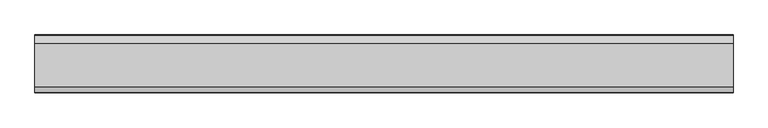
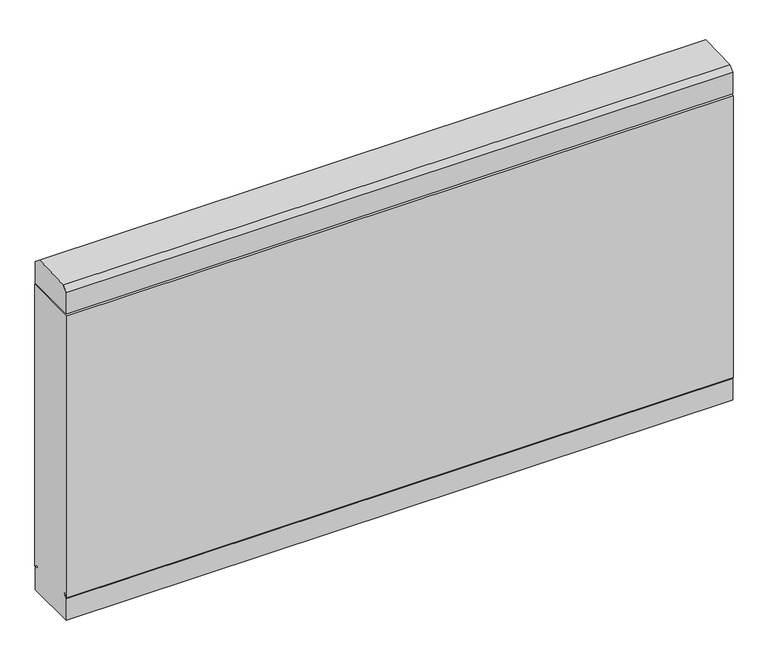
"""IFC4 building model written with IfcOpenShell, lengths in millimetres: proxy geometry, Generic Models 7:Generic Models 1:5:Generic Models 1:5 : Generic Models 7:Generic Models 1:337419:3 : Generic Models 7:Generic Models 1:5:Generic Models 1:5 : Generic Models 7:Generic Models 1:337419:311462."""

from ifc_helpers import new_model, si_unit, frame, origin, place, context, project, spatial, polyline, outline, extrude, source, transform, mapped, element, save


def generic_models_668826b1(model_context):
    return source(origin(), model_context, "Body", "SweptSolid", [
        extrude(outline(polyline([(-578799.0788841, 3616.325), (-578799.0788841, 2538.5457456), (-578812.2802009, 2549.6229657), (-578816.1067959, 2545.0626074), (-578801.8570091, 2533.1056165), (-578801.8570091, 2450.9015625), (-578996.3257591, 2450.9015625), (-578996.3257591, 2533.1056165), (-578982.0759722, 2545.0626074), (-578985.9025672, 2549.6229657), (-578999.1038841, 2538.5457456), (-578999.1038841, 3616.325), (-578799.0788841, 3616.325)])), frame((593776.1867239, 0.0, 0.0), z_axis=(1.0, 0.0, 0.0), x_axis=(0.0, 1.0, 0.0)), (0.0, 0.0, 1.0), 2406.65),
        extrude(outline(polyline([(-578801.8570091, 3622.278125), (-578996.3257591, 3622.278125), (-578996.3257591, 3704.482179), (-578977.2509963, 3720.4878054), (-578828.3268107, 3726.6929798), (-578801.8570091, 3704.482179), (-578801.8570091, 3622.278125)])), frame((593776.1867239, 0.0, 0.0), z_axis=(1.0, 0.0, 0.0), x_axis=(0.0, 1.0, 0.0)), (0.0, 0.0, 1.0), 2406.65),
    ])


if __name__ == "__main__":
    model = new_model("IFC4")
    model_context = context("Model", 3, world=origin())
    ifc_project = project(units=[si_unit("LENGTHUNIT", "METRE", prefix="MILLI")], contexts=[model_context])
    site = spatial("IfcSite", under=ifc_project)
    building = spatial("IfcBuilding", under=site)
    placement = place(None, origin())
    generic_models_shape = generic_models_668826b1(model_context)
    element("IfcBuildingElementProxy", 1, Name="Generic Models 7:Generic Models 1:5:Generic Models 1:5 : Generic Models 7:Generic Models 1:337419:3 : Generic Models 7:Generic Models 1:5:Generic Models 1:5 : Generic Models 7:Generic Models 1:337419:311462", ObjectType="Generic Models 7:Generic Models 1:5:Generic Models 1:5 : Generic Models 7:Generic Models 1:337419:3 : Generic Models 7:Generic Models 1:5:Generic Models 1:5 : Generic Models 7:Generic Models 1:337419:311462", at=placement, inside=building, context=model_context, shape_type="MappedRepresentation", body=[
        mapped(generic_models_shape, transform((0.0, 0.0, 0.0), x_axis=(1.0, 0.0, 0.0), y_axis=(0.0, 1.0, 0.0), z_axis=(0.0, 0.0, 1.0))),
    ])
    save(model, "model.ifc")

# Revit data of these elements
# Type "Generic Models 7:Generic Models 1:5:Generic Models 1:5 : Generic Models 7:Generic Models 1:337419:3 : Generic Models 7:Generic Models 1:5:Generic Models 1:5 : Generic Models 7:Generic Models 1:337419:311462"
#   NameOverride = "Generic Models 7:Generic Models 1:5:Generic Models 1:5 : Generic Models 7:Generic Models 1:337419:311462"
#   ObjectTypeOverride = "Generic Models 1:5 : Generic Models 7:Generic Models 1:337419"
#   Reference = "Generic Models 1"
#   Tag = "311462"
# Element 1 (IfcBuildingElementProxy, "Generic Models 7:Generic Models 1:5:Generic Models 1:5 : Generic Models 7:Generic Models 1:337419:3 : Generic Models 7:Generic Models 1:5:Generic Models 1:5 : Generic Models 7:Generic Models 1:337419:311462")
#   Materials on its faces: "SIMPLE SAVER INSULATION WITH LINER - COLOR: BLACK"
# Materials
#   "SIMPLE SAVER INSULATION WITH LINER - COLOR: BLACK": class "Unassigned", colour RGB 158 92 175, transparency 0, Cost = 0
